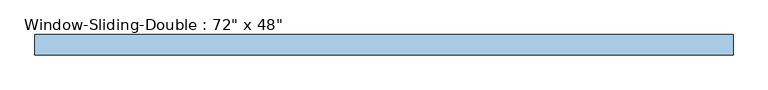
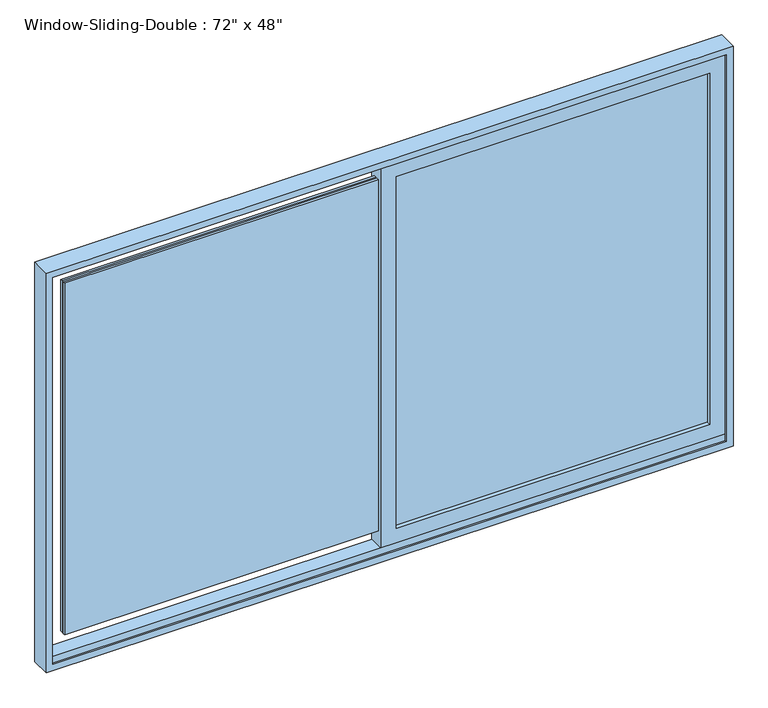
"""IFC4 building model written with IfcOpenShell, lengths in millimetres: window geometry."""

from ifc_helpers import new_model, si_unit, frame, origin, place, context, project, spatial, polyline, outline, extrude, faceted_brep, source, transform, mapped, element, save


def window_3387cd60(model_context):
    return source(origin(), model_context, "Body", "SolidModel", [
        faceted_brep([(-990.6, -10.16, 914.4), (-990.6, 46.99, 914.4), (990.6, 46.99, 914.4), (990.6, -10.16, 914.4), (-949.6778905, 46.99, 2092.6778905), (-949.6778905, 40.64, 2092.6778905), (-949.6778905, 40.64, 952.5), (-949.6778905, 40.64, 933.45), (-949.6778905, 46.99, 933.45), (949.6778905, 40.64, 2092.6778905), (949.6778905, 40.64, 952.5), (971.55, 40.64, 952.5), (971.55, 40.64, 2114.55), (-971.55, 40.64, 2114.55), (-971.55, 40.64, 952.5), (-971.55, -10.16, 2114.55), (-971.55, -10.16, 933.45), (-971.55, -3.81, 933.45), (-971.55, -3.81, 952.5), (990.6, -10.16, 2133.6), (-990.6, -10.16, 2133.6), (971.55, -10.16, 2114.55), (971.55, -10.16, 933.45), (-990.6, 46.99, 2133.6), (990.6, 46.99, 2133.6), (949.6778905, 46.99, 933.45), (949.6778905, 46.99, 2092.6778905), (949.6778905, 40.64, 933.45), (971.55, -3.81, 952.5), (971.55, -3.81, 933.45)], [[[0, 1, 2, 3]], [[4, 5, 6, 7, 8]], [[5, 9, 10, 11, 12, 13, 14, 6]], [[13, 15, 16, 17, 18, 14]], [[0, 3, 19, 20], [21, 22, 16, 15]], [[23, 1, 0, 20]], [[2, 1, 23, 24], [4, 8, 25, 26]], [[5, 4, 26, 9]], [[13, 12, 21, 15]], [[20, 19, 24, 23]], [[9, 26, 25, 27, 10]], [[21, 12, 11, 28, 29, 22]], [[19, 3, 2, 24]], [[7, 27, 25, 8]], [[27, 7, 6, 10]], [[10, 6, 14, 18, 28, 11]], [[28, 18, 17, 29]], [[16, 22, 29, 17]]]),
        extrude(outline(polyline([(927.1, 27.94), (927.1, 21.59), (22.225, 21.59), (22.225, 27.94), (927.1, 27.94)])), frame((0.0, 0.0, 996.95), z_axis=(0.0, 0.0, 1.0), x_axis=(1.0, 0.0, 0.0)), (0.0, 0.0, 1.0), 1073.15),
        extrude(outline(polyline([(927.1, 15.24), (927.1, 8.89), (22.225, 8.89), (22.225, 15.24), (927.1, 15.24)])), frame((0.0, 0.0, 996.95), z_axis=(0.0, 0.0, 1.0), x_axis=(1.0, 0.0, 0.0)), (0.0, 0.0, 1.0), 1073.15),
        extrude(outline(polyline([(-22.225, 27.94), (-22.225, 21.59), (-927.1, 21.59), (-927.1, 27.94), (-22.225, 27.94)])), frame((0.0, 0.0, 996.95), z_axis=(0.0, 0.0, 1.0), x_axis=(1.0, 0.0, 0.0)), (0.0, 0.0, 1.0), 1073.15),
        extrude(outline(polyline([(-22.225, 15.24), (-22.225, 8.89), (-927.1, 8.89), (-927.1, 15.24), (-22.225, 15.24)])), frame((0.0, 0.0, 996.95), z_axis=(0.0, 0.0, 1.0), x_axis=(1.0, 0.0, 0.0)), (0.0, 0.0, 1.0), 1073.15),
        extrude(outline(polyline([(952.5, 971.55), (2114.55, 971.55), (2114.55, -22.225), (952.5, -22.225), (952.5, 971.55)]), holes=[polyline([(996.95, 22.225), (2070.1, 22.225), (2070.1, 927.1), (996.95, 927.1), (996.95, 22.225)])]), frame((0.0, -3.81, 0.0), z_axis=(0.0, 1.0, 0.0), x_axis=(0.0, 0.0, 1.0)), (0.0, 0.0, 1.0), 44.45),
    ])


if __name__ == "__main__":
    model = new_model("IFC4")
    model_context = context("Model", 3, world=origin())
    ifc_project = project(units=[si_unit("LENGTHUNIT", "METRE", prefix="MILLI")], contexts=[model_context])
    site = spatial("IfcSite", under=ifc_project)
    building = spatial("IfcBuilding", under=site)
    placement = place(None, origin())
    window_shape = window_3387cd60(model_context)
    element("IfcWindow", 1, ObjectType="Window-Sliding-Double : 72\" x 48\"", at=placement, inside=building, context=model_context, shape_type="MappedRepresentation", body=[
        mapped(window_shape, transform((0.0, 0.0, 0.0), x_axis=(1.0, 0.0, 0.0), y_axis=(0.0, 1.0, 0.0), z_axis=(0.0, 0.0, 1.0))),
    ])
    save(model, "model.ifc")

# Revit data of these elements
# Type "Window-Sliding-Double : 72\" x 48\""
#   Type Mark = "23"
#   Fire Rating = "0.5h"
#   Assembly Code = "B2020100"
#   Analytic Construction = "Double glazing - domestic"
#   Window Inset [instance default] = 0' - 0"
#   Wall Thickness [instance default] = 0' - 6"
#   Visual Light Transmittance = 0.81
#   Thermal Resistance (R) = 1.8146 (h·ft²·°F)/BTU
#   Solar Heat Gain Coefficient = 0.76
#   Muntin Width = 2' - 11 5/8"
#   Muntin Height = 3' - 6 1/4"
#   Interior Wall Closure [instance default] = 0' - 2 3/4"
#   Heat Transfer Coefficient (U) = 0.5511 BTU/(h·ft²·°F)
#   Frame Extension [instance default] = 0' - 0 1/4"
#   Exterior Wall Closure [instance default] = 0' - 1 1/4"
#   Rough Width = 6' - 6 1/2"
#   Rough Height = 4' - 0 1/2"
#   Height = 4' - 0"
#   Extension Jamb [instance default] = 0' - 2 3/4"
#   Default Sill Height = 3' - 0"
#   Width = 6' - 6"
#   Interior Trim Visibility [instance default] = yes
#   Indicator Visibility [instance default] = yes
#   Exterior Trim Visibility [instance default] = yes
#   Muntin Visibility = yes
#   Extension Jamb Visibility [instance default] = yes
#   Muntin Pattern = Muntin Pattern_2x2 : Muntin Pattern_2x2
#   Interior Trim Material = Wood - Stained
#   Interior Trim = Trim-Window-Interior-Flat : Picture Frame
#   Interior Frame Material = Wood - Stained
#   Glass Panel Material = Glass
#   Exterior Trim Material = Clad - White
#   Exterior Trim = Trim-Window-Exterior-Flat : with Sill
#   Exterior Frame Material = Clad - White
#   Wall Closure = (empty or 0)
# Element 1 (IfcWindow, "Window-Sliding-Double : 72\" x 48\"")
#   Wall Thickness = 0' - 2 1/2"
#   Extension Jamb = 0' - 1"
#   Extension Jamb Visibility = no
#   Materials on its faces: "Glass", "Wood - Stained", "Clad - White"
# Materials
#   "Wood - Stained": class "Wood", colour RGB 224 178 126, transparency 0, Cost = 0
#   "Glass": class "Glass", colour RGB 0 128 192, transparency 0.75, Description = "Soda Lime Glass", Cost = 0
#   "Clad - White": class "Wood", colour RGB 242 242 238, transparency 0, Cost = 0
